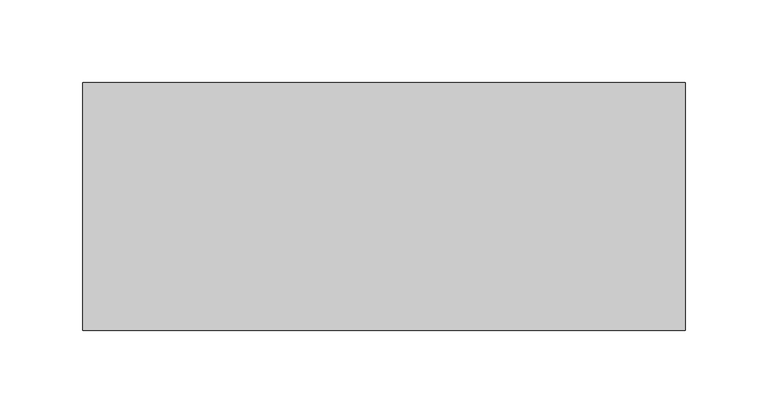
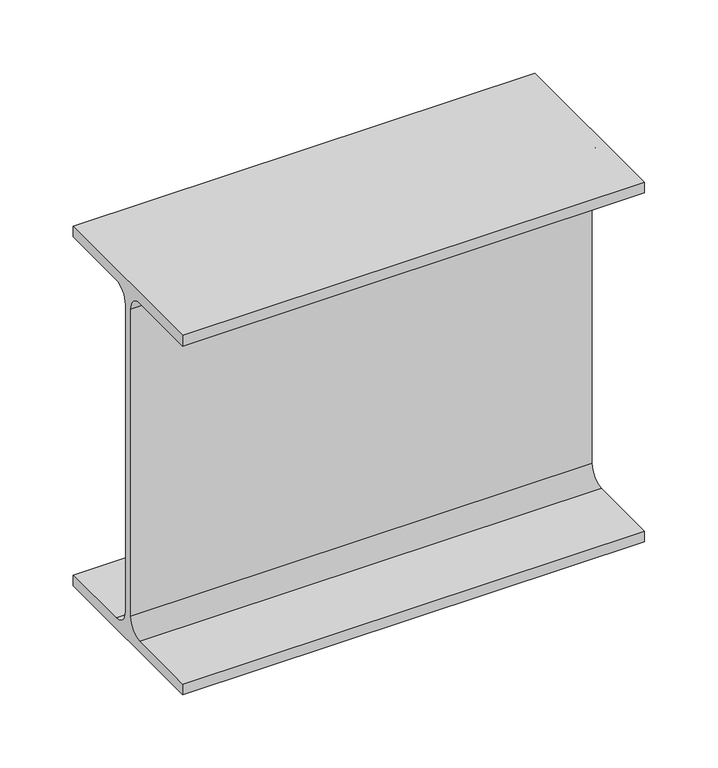
"""IFC4 building model written with IfcOpenShell, lengths in millimetres: beam geometry, 0912_Steel Framing_H-KSD3502 : H_SB_ASB_H-300x150x6.5x9."""

import ifcopenshell
import ifcopenshell.guid

model = None  # the IFC model being written
_history = None  # IfcOwnerHistory: only IFC2X3 demands one
_inside = {}  # id of a spatial element -> (the spatial element, [elements in it])
_under = {}  # id of a project, library or spatial element -> (it, [spatial elements below it])
_declared = {}  # id of a project -> (the project, [libraries it declares])
_typed = {}  # id of a type object -> (the type object, [elements of that type])
_made_of = {}  # id of a material, layer set ... -> (it, [elements and type objects made of it])


def new_model(schema):
    """Start an empty IFC model of exactly this schema.

    Asked for "IFC4X3", IfcOpenShell would pick the latest addendum, in which some entities
    have other attributes; the version numbers below select the first issue.
    IFC2X3 requires an IfcOwnerHistory on every rooted entity: one is made here for all.
    """
    global model, _history
    if schema == "IFC4X3":
        model = ifcopenshell.file(schema_version=(4, 3, 0, 0))
    else:
        model = ifcopenshell.file(schema=schema)
    _inside.clear()
    _under.clear()
    _declared.clear()
    _typed.clear()
    _made_of.clear()
    _history = None
    if model.schema == "IFC2X3":
        org = make("IfcOrganization", Name="unknown")
        user = make(
            "IfcPersonAndOrganization",
            ThePerson=make("IfcPerson", FamilyName="unknown"),
            TheOrganization=org,
        )
        app = make(
            "IfcApplication",
            ApplicationDeveloper=org,
            Version="unknown",
            ApplicationFullName="unknown",
            ApplicationIdentifier="unknown",
        )
        _history = make(
            "IfcOwnerHistory",
            OwningUser=user,
            OwningApplication=app,
            ChangeAction="ADDED",
            CreationDate=0,
        )
    return model


def make(cls, **values):
    """One entity of the class cls with the attributes given. An attribute that is None is left unset."""
    return model.create_entity(
        cls, **{name: value for name, value in values.items() if value is not None}
    )


def rooted(cls, **values):
    """An entity with a GlobalId (a new one), such as an element, a storey or a relation."""
    return make(cls, GlobalId=ifcopenshell.guid.new(), OwnerHistory=_history, **values)


def si_unit(unit_type, name, prefix=None):
    """IfcSIUnit, for example si_unit("LENGTHUNIT", "METRE", prefix="MILLI")."""
    return make("IfcSIUnit", UnitType=unit_type, Prefix=prefix, Name=name)


def assignment(units):
    """IfcUnitAssignment: the units of a project."""
    return None if units is None else make("IfcUnitAssignment", Units=units)


def point(xyz):
    """IfcCartesianPoint."""
    return None if xyz is None else make("IfcCartesianPoint", Coordinates=xyz)


def direction(xyz):
    """IfcDirection."""
    return None if xyz is None else make("IfcDirection", DirectionRatios=xyz)


def frame(location, z_axis=None, x_axis=None):
    """IfcAxis2Placement3D, a coordinate frame: its origin and axes. An axis left out is left unset."""
    return make(
        "IfcAxis2Placement3D",
        Location=point(location),
        Axis=direction(z_axis),
        RefDirection=direction(x_axis),
    )


def frame_2d(location, x_axis=None):
    """IfcAxis2Placement2D, a coordinate frame in the plane: its origin and x axis."""
    return make(
        "IfcAxis2Placement2D", Location=point(location), RefDirection=direction(x_axis)
    )


def origin():
    """The frame at (0, 0, 0) with its axes left unset."""
    return frame((0.0, 0.0, 0.0))


def place(relative_to, where):
    """IfcLocalPlacement: puts the frame where relative to a parent placement (None: the world)."""
    return make(
        "IfcLocalPlacement", PlacementRelTo=relative_to, RelativePlacement=where
    )


def context(
    kind, dimensions, precision=None, world=None, true_north=None, identifier=None
):
    """IfcGeometricRepresentationContext, for example the 3D "Model" context."""
    return make(
        "IfcGeometricRepresentationContext",
        ContextIdentifier=identifier,
        ContextType=kind,
        CoordinateSpaceDimension=dimensions,
        Precision=precision,
        WorldCoordinateSystem=world,
        TrueNorth=true_north,
    )


def project(units=None, contexts=None):
    """IfcProject with its units and contexts."""
    return rooted(
        "IfcProject",
        Name="project",
        RepresentationContexts=contexts,
        UnitsInContext=assignment(units),
    )


def spatial(cls, under=None, at=None, **own):
    """A site, building, storey or space (cls), placed at a placement, below another one or the project."""
    s = rooted(cls, ObjectPlacement=at, **own)
    if under is not None:
        _under.setdefault(under.id(), (under, []))[1].append(s)
    return s


def polyline(points):
    """IfcPolyline through the points."""
    return make("IfcPolyline", Points=[point(p) for p in points])


def circle_curve(where, radius):
    """IfcCircle in the frame where."""
    return make("IfcCircle", Position=where, Radius=radius)


def trimmed(basis, trim1, trim2, sense, master):
    """IfcTrimmedCurve: the piece of a basis curve between two trims."""
    return make(
        "IfcTrimmedCurve",
        BasisCurve=basis,
        Trim1=trim1,
        Trim2=trim2,
        SenseAgreement=sense,
        MasterRepresentation=master,
    )


def segment(curve, same_sense, transition):
    """IfcCompositeCurveSegment."""
    return make(
        "IfcCompositeCurveSegment",
        Transition=transition,
        SameSense=same_sense,
        ParentCurve=curve,
    )


def composite_curve(segments, self_intersect=None):
    """IfcCompositeCurve: segments joined end to end."""
    return make("IfcCompositeCurve", Segments=segments, SelfIntersect=self_intersect)


def outline(outer, holes=None, kind="AREA"):
    """IfcArbitraryClosedProfileDef: a profile drawn as a closed curve; with holes, ...WithVoids."""
    if holes is None:
        return make("IfcArbitraryClosedProfileDef", ProfileType=kind, OuterCurve=outer)
    return make(
        "IfcArbitraryProfileDefWithVoids",
        ProfileType=kind,
        OuterCurve=outer,
        InnerCurves=holes,
    )


def extrude(swept, where, along, depth):
    """IfcExtrudedAreaSolid: the profile swept, set in the frame where, extruded along a direction by depth."""
    return make(
        "IfcExtrudedAreaSolid",
        SweptArea=swept,
        Position=where,
        ExtrudedDirection=direction(along),
        Depth=depth,
    )


def shape(context_of_items, identifier, shape_type, items):
    """IfcShapeRepresentation: the items that make up one representation, for example the "Body"."""
    return make(
        "IfcShapeRepresentation",
        ContextOfItems=context_of_items,
        RepresentationIdentifier=identifier,
        RepresentationType=shape_type,
        Items=items,
    )


def source(mapping_origin, context_of_items, identifier, shape_type, items):
    """IfcRepresentationMap: a shape defined once, which mapped items show again and again."""
    return make(
        "IfcRepresentationMap",
        MappingOrigin=mapping_origin,
        MappedRepresentation=shape(context_of_items, identifier, shape_type, items),
    )


def transform(
    local_origin,
    x_axis=None,
    y_axis=None,
    z_axis=None,
    scale=None,
    scale2=None,
    scale3=None,
    uniform=True,
):
    """IfcCartesianTransformationOperator3D, or its non-uniform kind. x_axis, y_axis, z_axis: its Axis1, 2, 3."""
    if uniform:
        return make(
            "IfcCartesianTransformationOperator3D",
            Axis1=direction(x_axis),
            Axis2=direction(y_axis),
            LocalOrigin=point(local_origin),
            Scale=scale,
            Axis3=direction(z_axis),
        )
    return make(
        "IfcCartesianTransformationOperator3DnonUniform",
        Axis1=direction(x_axis),
        Axis2=direction(y_axis),
        LocalOrigin=point(local_origin),
        Scale=scale,
        Axis3=direction(z_axis),
        Scale2=scale2,
        Scale3=scale3,
    )


def mapped(mapping_source, mapping_target):
    """IfcMappedItem: shows the shape of a source again, moved by a transform."""
    return make(
        "IfcMappedItem", MappingSource=mapping_source, MappingTarget=mapping_target
    )


def made_of(thing, what):
    """Note that an element or type object is made of a material, layer set ...; save() writes the relation."""
    if what is not None:
        _made_of.setdefault(what.id(), (what, []))[1].append(thing)
    return thing


def element(
    cls,
    number,
    at=None,
    inside=None,
    cuts=None,
    type_object=None,
    material=None,
    context=None,
    identifier="Body",
    shape_type=None,
    held_by="IfcProductDefinitionShape",
    body=None,
    shapes=None,
    **own,
):
    """One element of the class cls, such as IfcWall. Its Tag is "e" and its number.

    at: its placement. inside: the storey or other place that contains it. cuts: it is an
    opening in that element (IfcRelVoidsElement). A single representation is given by context,
    identifier, shape_type and body (its items); several are given by shapes. held_by: the class
    of the entity that holds the representations. save() writes the other relations.
    """
    e = rooted(cls, Tag="e%d" % number, ObjectPlacement=at, **own)
    if body is not None:
        shapes = [shape(context, identifier, shape_type, body)]
    if shapes is not None:
        e.Representation = make(held_by, Representations=shapes)
    if inside is not None:
        _inside.setdefault(inside.id(), (inside, []))[1].append(e)
    if cuts is not None:
        rooted(
            "IfcRelVoidsElement", RelatingBuildingElement=cuts, RelatedOpeningElement=e
        )
    if type_object is not None:
        _typed.setdefault(type_object.id(), (type_object, []))[1].append(e)
    return made_of(e, material)


def aggregate(whole, parts):
    """IfcRelAggregates: a whole, such as a stair, and the parts it consists of."""
    return rooted("IfcRelAggregates", RelatingObject=whole, RelatedObjects=parts)


def save(model, path):
    """Write the relations noted so far, then the file.

    IfcRelAggregates (storeys below a building ...), IfcRelContainedInSpatialStructure (elements
    in a storey), IfcRelDefinesByType, IfcRelAssociatesMaterial and IfcRelDeclares: one each for
    every whole, place, type object, material and project.
    """
    for whole, parts in _under.values():
        aggregate(whole, parts)
    for where, things in _inside.values():
        rooted(
            "IfcRelContainedInSpatialStructure",
            RelatedElements=things,
            RelatingStructure=where,
        )
    for kind, things in _typed.values():
        rooted("IfcRelDefinesByType", RelatedObjects=things, RelatingType=kind)
    for what, things in _made_of.values():
        rooted("IfcRelAssociatesMaterial", RelatedObjects=things, RelatingMaterial=what)
    for by, libraries in _declared.values():
        rooted("IfcRelDeclares", RelatingContext=by, RelatedDefinitions=libraries)
    model.write(path)


def beam_5b55ed88(model_context):
    return source(origin(), model_context, "Body", "SweptSolid", [
        extrude(outline(composite_curve([segment(polyline([(75.0, -141.0), (75.0, -150.0), (-75.0, -150.0), (-75.0, -141.0), (-16.25, -141.0)]), True, "CONTINUOUS"), segment(trimmed(circle_curve(frame_2d((-16.25, -128.0)), 13.0), [point((-16.25, -141.0))], [point((-3.25, -128.0))], True, "CARTESIAN"), True, "CONTINUOUS"), segment(polyline([(-3.25, -128.0), (-3.25, 128.0)]), True, "CONTINUOUS"), segment(trimmed(circle_curve(frame_2d((-16.25, 128.0)), 13.0), [point((-3.25, 128.0))], [point((-16.25, 141.0))], True, "CARTESIAN"), True, "CONTINUOUS"), segment(polyline([(-16.25, 141.0), (-75.0, 141.0), (-75.0, 150.0), (75.0, 150.0), (75.0, 141.0), (16.25, 141.0)]), True, "CONTINUOUS"), segment(trimmed(circle_curve(frame_2d((16.25, 128.0)), 13.0), [point((16.25, 141.0))], [point((3.25, 128.0))], True, "CARTESIAN"), True, "CONTINUOUS"), segment(polyline([(3.25, 128.0), (3.25, -128.0)]), True, "CONTINUOUS"), segment(trimmed(circle_curve(frame_2d((16.25, -128.0)), 13.0), [point((3.25, -128.0))], [point((16.25, -141.0))], True, "CARTESIAN"), True, "CONTINUOUS"), segment(polyline([(16.25, -141.0), (75.0, -141.0)]), True, "CONTINUOUS")], self_intersect=False)), frame((-82.3, 0.0, 0.0), z_axis=(1.0, 0.0, 0.0), x_axis=(0.0, 1.0, 0.0)), (0.0, 0.0, 1.0), 364.6),
    ])


if __name__ == "__main__":
    model = new_model("IFC4")
    model_context = context("Model", 3, world=origin())
    ifc_project = project(units=[si_unit("LENGTHUNIT", "METRE", prefix="MILLI")], contexts=[model_context])
    site = spatial("IfcSite", under=ifc_project)
    building = spatial("IfcBuilding", under=site)
    placement = place(None, origin())
    beam_shape = beam_5b55ed88(model_context)
    element("IfcBeam", 1, ObjectType="0912_Steel Framing_H-KSD3502 : H_SB_ASB_H-300x150x6.5x9", at=placement, inside=building, context=model_context, shape_type="MappedRepresentation", body=[
        mapped(beam_shape, transform((0.0, 0.0, 0.0), x_axis=(1.0, 0.0, 0.0), y_axis=(0.0, 1.0, 0.0), z_axis=(0.0, 0.0, 1.0))),
    ])
    save(model, "model.ifc")

# Revit data of these elements
# Type "0912_Steel Framing_H-KSD3502 : H_SB_ASB_H-300x150x6.5x9"
#   H_WM Code_1 = "S01AA002-00001 | Main Steel Structure Fabrication Work | Shelter/Building | Medium Steel - Standard (90KG/M>Weight≥30KG/M) | Material: (   )"
#   H_WM Code_2 = "S03AA028-00001 | Main Steel Structure Erection Work | Shelter/Building | Medium Steel (90KG/M>Weight≥30KG/M) | Material: (   )"
#   H_WM Code_3 = "S01AA010-00001 | Main Steel Structure Fabrication Work | Shelter/Building | Steel Painting/Coating | for Non-Fireproofed Steel Surface, Surface Preparation, Primer, Second & Final Coat | Material: (   )"
#   H_Q'ty Cal Type Tag = "SB-Q2"
#   Width = 15.0 cm
#   Web Thickness = 0.65 cm
#   Web Fillet = 1.3 cm
#   Warping Constant = 107000.0 cm⁶
#   W = 0
#   Torsional Moment of Inertia = 9.9539 cm⁴
#   Section Area = 46.78 cm²
#   Plastic Modulus weak axis = 105.0 cm³
#   Plastic Modulus strong axis = 542.0 cm³
#   Perimeter = 1.17 m²/m
#   Nominal Weight = 36.70 kgf/m
#   Moment of Inertia weak axis = 508.00 cm⁴
#   Moment of Inertia strong axis = 7210.00 cm⁴
#   Height = 30.0 cm
#   Flange Thickness = 0.9 cm
#   Elastic Modulus weak axis = 67.7 cm³
#   Elastic Modulus strong axis = 481.0 cm³
#   Centroid Vertical = 15.0 cm
#   Centroid Horizontal = 7.5 cm
#   Ix = 72100000
#   Length [instance default] = 1.5240 m
#   Zx = 542000
#   b = 0.1500 m
#   h = 0.3000 m
#   r = 0.0130 m
#   s = 0.0065 m
#   t = 0.0090 m
#   A = 0.004678 m²
#   Structural Material [instance default] = Steel, 45-345
#   Assembly Code = ""
# Element 1 (IfcBeam, "0912_Steel Framing_H-KSD3502 : H_SB_ASB_H-300x150x6.5x9")
#   Structural Material = none
# Materials
#   "Steel, 45-345": class "Metal", colour RGB 189 187 185, transparency 0, Description = "Steel 345 MPa", Cost = 0
